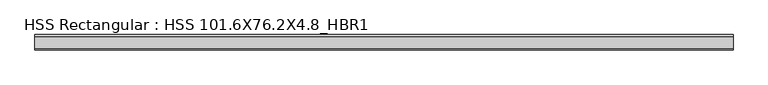
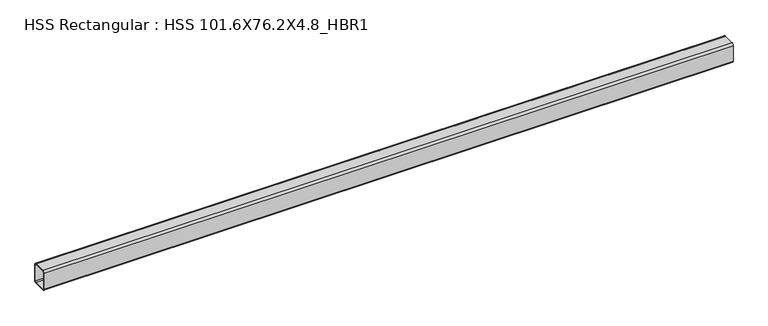
"""IFC4 building model written with IfcOpenShell, lengths in millimetres: beam geometry, HSS Rectangular : HSS 101.6X76.2X4.8_HBR1."""

from ifc_helpers import new_model, si_unit, point, frame, frame_2d, origin, place, context, project, spatial, polyline, circle_curve, trimmed, segment, composite_curve, outline, extrude, source, transform, mapped, element, save


def hss_rectangular_hss_101_6x76_2x4_8_hbr1_fbc9fe96(model_context):
    return source(origin(), model_context, "Body", "SweptSolid", [
        extrude(outline(composite_curve([segment(polyline([(38.1, 41.275), (38.1, -41.275)]), True, "CONTINUOUS"), segment(trimmed(circle_curve(frame_2d((28.575, -41.275)), 9.525), [point((38.1, -41.275))], [point((28.575, -50.8))], False, "CARTESIAN"), True, "CONTINUOUS"), segment(polyline([(28.575, -50.8), (-28.575, -50.8)]), True, "CONTINUOUS"), segment(trimmed(circle_curve(frame_2d((-28.575, -41.275)), 9.525), [point((-28.575, -50.8))], [point((-38.1, -41.275))], False, "CARTESIAN"), True, "CONTINUOUS"), segment(polyline([(-38.1, -41.275), (-38.1, 41.275)]), True, "CONTINUOUS"), segment(trimmed(circle_curve(frame_2d((-28.575, 41.275)), 9.525), [point((-38.1, 41.275))], [point((-28.575, 50.8))], False, "CARTESIAN"), True, "CONTINUOUS"), segment(polyline([(-28.575, 50.8), (28.575, 50.8)]), True, "CONTINUOUS"), segment(trimmed(circle_curve(frame_2d((28.575, 41.275)), 9.525), [point((28.575, 50.8))], [point((38.1, 41.275))], False, "CARTESIAN"), True, "CONTINUOUS")], self_intersect=False), holes=[composite_curve([segment(trimmed(circle_curve(frame_2d((-28.575, 41.275)), 4.7625), [point((-28.575, 46.0375))], [point((-33.3375, 41.275))], True, "CARTESIAN"), True, "CONTINUOUS"), segment(polyline([(-33.3375, 41.275), (-33.3375, -41.275)]), True, "CONTINUOUS"), segment(trimmed(circle_curve(frame_2d((-28.575, -41.275)), 4.7625), [point((-33.3375, -41.275))], [point((-28.575, -46.0375))], True, "CARTESIAN"), True, "CONTINUOUS"), segment(polyline([(-28.575, -46.0375), (28.575, -46.0375)]), True, "CONTINUOUS"), segment(trimmed(circle_curve(frame_2d((28.575, -41.275)), 4.7625), [point((28.575, -46.0375))], [point((33.3375, -41.275))], True, "CARTESIAN"), True, "CONTINUOUS"), segment(polyline([(33.3375, -41.275), (33.3375, 41.275)]), True, "CONTINUOUS"), segment(trimmed(circle_curve(frame_2d((28.575, 41.275)), 4.7625), [point((33.3375, 41.275))], [point((28.575, 46.0375))], True, "CARTESIAN"), True, "CONTINUOUS"), segment(polyline([(28.575, 46.0375), (-28.575, 46.0375)]), True, "CONTINUOUS")], self_intersect=False)]), frame((-1606.9719751, 0.0, 0.0), z_axis=(1.0, 0.0, 0.0), x_axis=(0.0, 1.0, 0.0)), (0.0, 0.0, 1.0), 3417.8948165),
    ])


if __name__ == "__main__":
    model = new_model("IFC4")
    model_context = context("Model", 3, world=origin())
    ifc_project = project(units=[si_unit("LENGTHUNIT", "METRE", prefix="MILLI")], contexts=[model_context])
    site = spatial("IfcSite", under=ifc_project)
    building = spatial("IfcBuilding", under=site)
    placement = place(None, origin())
    hss_rectangular_hss_101_6x76_2x4_8_hbr1_shape = hss_rectangular_hss_101_6x76_2x4_8_hbr1_fbc9fe96(model_context)
    element("IfcBeam", 1, ObjectType="HSS Rectangular : HSS 101.6X76.2X4.8_HBR1", at=placement, inside=building, context=model_context, shape_type="MappedRepresentation", body=[
        mapped(hss_rectangular_hss_101_6x76_2x4_8_hbr1_shape, transform((0.0, 0.0, 0.0), x_axis=(1.0, 0.0, 0.0), y_axis=(0.0, 1.0, 0.0), z_axis=(0.0, 0.0, 1.0))),
    ])
    save(model, "model.ifc")

# Revit data of these elements
# Type "HSS Rectangular : HSS 101.6X76.2X4.8_HBR1"
#   Section Name Key = "HSS 4X3X3/16"
#   Assembly Code = "B10"
#   Width = 7.62 cm
#   Wall Nominal Thickness = 0.4763 cm
#   Wall Design Thickness = 0.442 cm
#   Torsional Moment of Inertia = 260.561 cm⁴
#   Torsional Modulus = 61.2876 cm³
#   Section Area = 14.4516 cm²
#   Plastic Modulus weak axis = 40.3122 cm³
#   Plastic Modulus strong axis = 49.1612 cm³
#   Perimeter = 0.881482 m²/m
#   Outer Fillet = 0.9525 cm
#   Nominal Weight = 12.1285 kgf/m
#   Moment of Inertia weak axis = 131.529 cm⁴
#   Moment of Inertia strong axis = 205.202 cm⁴
#   Inner Fillet = 0.4763 cm
#   Height = 10.16 cm
#   Elastic Modulus weak axis = 34.4128 cm³
#   Elastic Modulus strong axis = 40.476 cm³
#   Centroid Vertical = 5.08 cm
#   Centroid Horizontal = 3.81 cm
#   Length [instance default] = 1524 mm
#   Structural Material [instance default] = Steel ASTM A500, Grade B, Rectangular and Square
#   Principal Axes Angle = 0
# Element 1 (IfcBeam, "HSS Rectangular : HSS 101.6X76.2X4.8_HBR1")
#   Structural Material = Steel ASTM A992
#   Materials on its faces: "Steel ASTM A992"
# Materials
#   "Steel ASTM A500, Grade B, Rectangular and Square": class "Metal", colour RGB 199 199 199, transparency 0, Description = "Carbon steel", Cost = 0
#   "Steel ASTM A992": class "Metal", colour RGB 199 199 199, transparency 0, Description = "Structural steel 50ksi", Cost = 0
